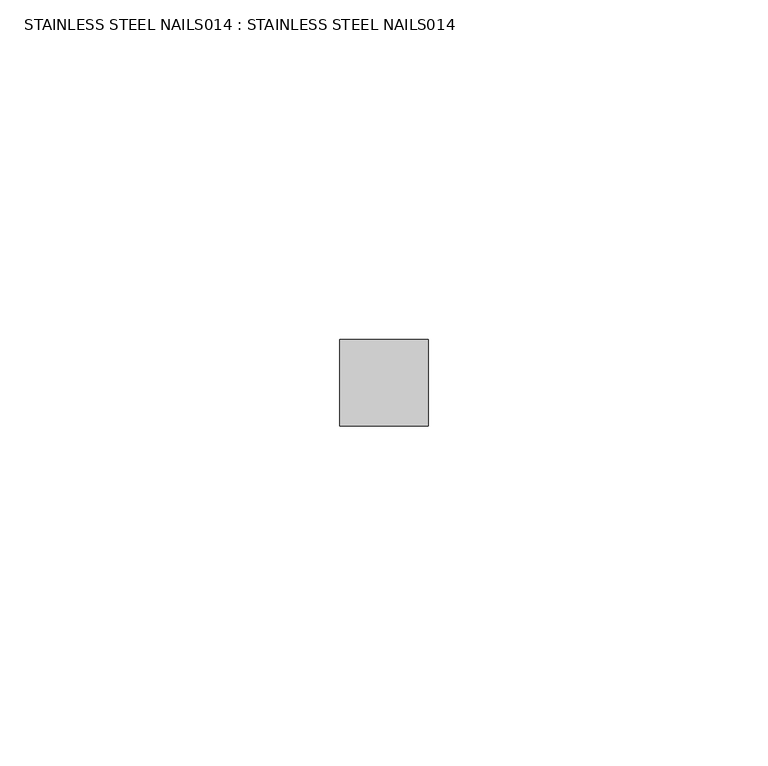
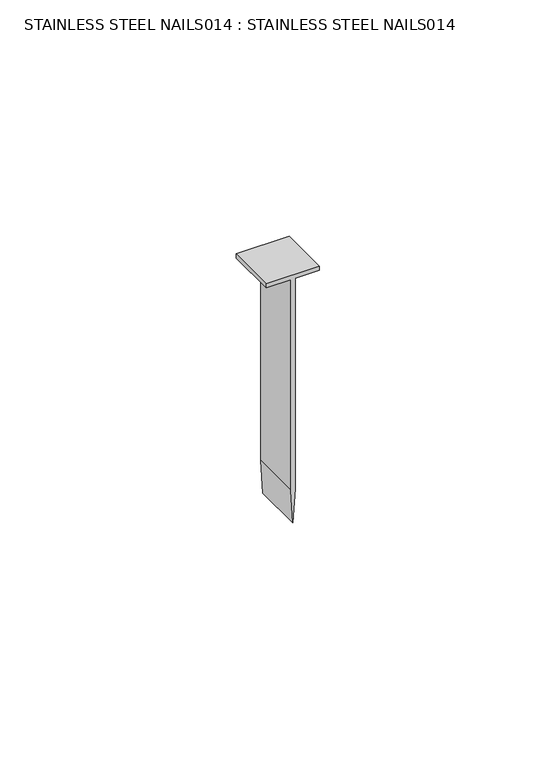
"""IFC4 building model written with IfcOpenShell, lengths in millimetres: proxy geometry, STAINLESS STEEL NAILS014 : STAINLESS STEEL NAILS014."""

from ifc_helpers import new_model, si_unit, frame, origin, place, context, project, spatial, polyline, outline, extrude, source, transform, mapped, element, save


def stainless_steel_nails014_stainless_steel_nails014_b48167de(model_context):
    return source(origin(), model_context, "Body", "SweptSolid", [
        extrude(outline(polyline([(40259.5998489, -4467.2441308), (40260.6830476, -4467.2441308), (40260.6830476, -4480.2425147), (40259.5998489, -4480.2425147), (40259.5998489, -4474.2849221), (40205.2729558, -4474.2849221), (40196.6073666, -4473.7433228), (40205.2729558, -4473.2017234), (40259.5998489, -4473.2017234), (40259.5998489, -4467.2441308)])), frame((0.0, 934.6593427, 0.0), z_axis=(0.0, 1.0, 0.0), x_axis=(0.0, 0.0, 1.0)), (0.0, 0.0, 1.0), 12.7),
    ])


if __name__ == "__main__":
    model = new_model("IFC4")
    model_context = context("Model", 3, world=origin())
    ifc_project = project(units=[si_unit("LENGTHUNIT", "METRE", prefix="MILLI")], contexts=[model_context])
    site = spatial("IfcSite", under=ifc_project)
    building = spatial("IfcBuilding", under=site)
    placement = place(None, origin())
    stainless_steel_nails014_stainless_steel_nails014_shape = stainless_steel_nails014_stainless_steel_nails014_b48167de(model_context)
    element("IfcBuildingElementProxy", 1, Name="STAINLESS STEEL NAILS014 : STAINLESS STEEL NAILS014", ObjectType="STAINLESS STEEL NAILS014 : STAINLESS STEEL NAILS014", at=placement, inside=building, context=model_context, shape_type="MappedRepresentation", body=[
        mapped(stainless_steel_nails014_stainless_steel_nails014_shape, transform((0.0, 0.0, 0.0), x_axis=(1.0, 0.0, 0.0), y_axis=(0.0, 1.0, 0.0), z_axis=(0.0, 0.0, 1.0))),
    ])
    save(model, "model.ifc")

# Revit data of these elements
# Type "STAINLESS STEEL NAILS014 : STAINLESS STEEL NAILS014"
#   NameOverride = "STAINLESS STEEL NAILS014"
# Element 1 (IfcBuildingElementProxy, "STAINLESS STEEL NAILS014 : STAINLESS STEEL NAILS014")
#   Materials on its faces: "1 3/4\" STAINLESS STEEL RINGSHANK 5D COMMON NAILS @ 4\" (101.6MM) O.C. FIRESTONE PROVIDED MAX., 1/2\" STAGGERED"
# Materials
#   "1 3/4\" STAINLESS STEEL RINGSHANK 5D COMMON NAILS @ 4\" (101.6MM) O.C. FIRESTONE PROVIDED MAX., 1/2\" STAGGERED": class "Unassigned", colour RGB 255 255 255, transparency 0
